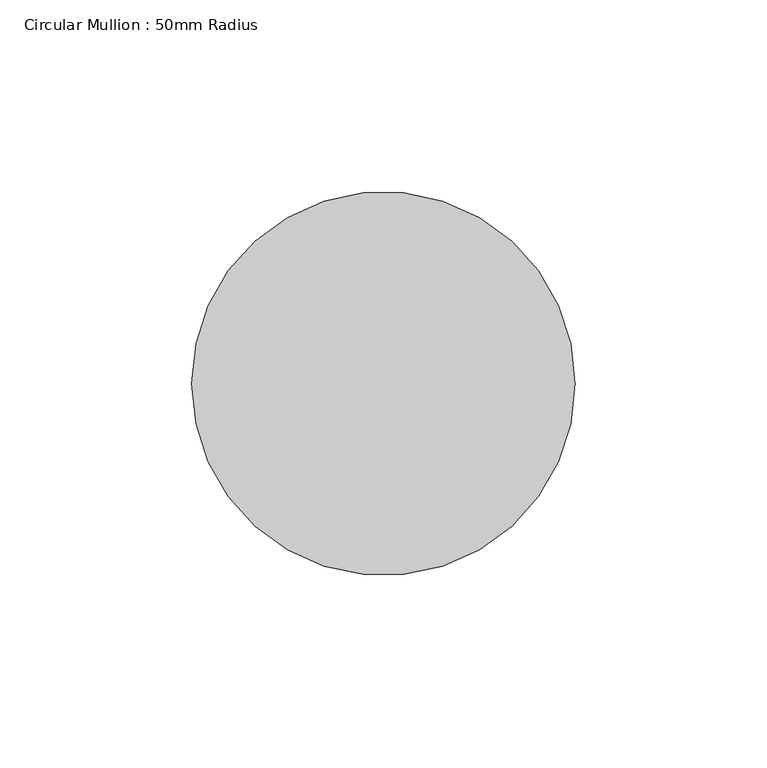
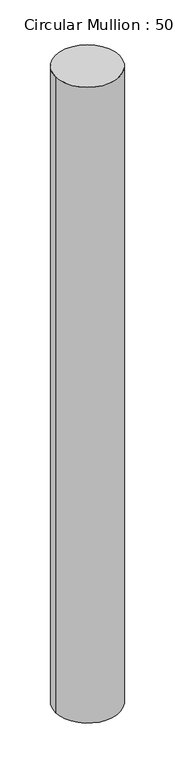
"""IFC4 building model written with IfcOpenShell, lengths in millimetres: member geometry, Circular Mullion : 50mm Radius."""

from ifc_helpers import new_model, si_unit, point, frame, origin, origin_2d, place, context, project, spatial, circle_curve, trimmed, segment, composite_curve, outline, extrude, source, transform, mapped, element, save


def circular_mullion_50mm_radius_c066c39f(model_context):
    return source(origin(), model_context, "Body", "SweptSolid", [
        extrude(outline(composite_curve([segment(trimmed(circle_curve(origin_2d(), 50.0), [point((50.0, 0.0))], [point((-50.0, 0.0))], False, "CARTESIAN"), True, "CONTINUOUS"), segment(trimmed(circle_curve(origin_2d(), 50.0), [point((-50.0, 0.0))], [point((50.0, 0.0))], False, "CARTESIAN"), True, "CONTINUOUS")], self_intersect=False)), frame((0.0, 0.0, -1047.3216576), z_axis=(0.0, 0.0, 1.0), x_axis=(1.0, 0.0, 0.0)), (0.0, 0.0, 1.0), 1047.3216576),
    ])


if __name__ == "__main__":
    model = new_model("IFC4")
    model_context = context("Model", 3, world=origin())
    ifc_project = project(units=[si_unit("LENGTHUNIT", "METRE", prefix="MILLI")], contexts=[model_context])
    site = spatial("IfcSite", under=ifc_project)
    building = spatial("IfcBuilding", under=site)
    placement = place(None, origin())
    circular_mullion_50mm_radius_shape = circular_mullion_50mm_radius_c066c39f(model_context)
    element("IfcMember", 1, ObjectType="Circular Mullion : 50mm Radius", at=placement, inside=building, context=model_context, shape_type="MappedRepresentation", body=[
        mapped(circular_mullion_50mm_radius_shape, transform((0.0, 0.0, 0.0), x_axis=(1.0, 0.0, 0.0), y_axis=(0.0, 1.0, 0.0), z_axis=(0.0, 0.0, 1.0))),
    ])
    save(model, "model.ifc")

# Revit data of these elements
# Type "Circular Mullion : 50mm Radius"
#   built-in parameter 1007350 = 0.164042 (stored number, unit not read)
# Element 1 (IfcMember, "Circular Mullion : 50mm Radius")
#   Materials on its faces: "Aluminium"
# Materials
#   "Aluminium": class "Metal", colour RGB 247 247 247, transparency 0, Description = "Aluminium 6061", Cost = 0
